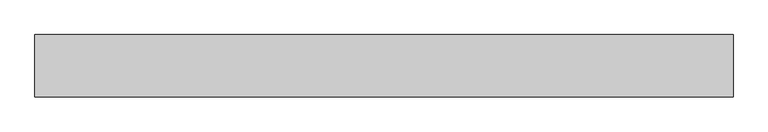
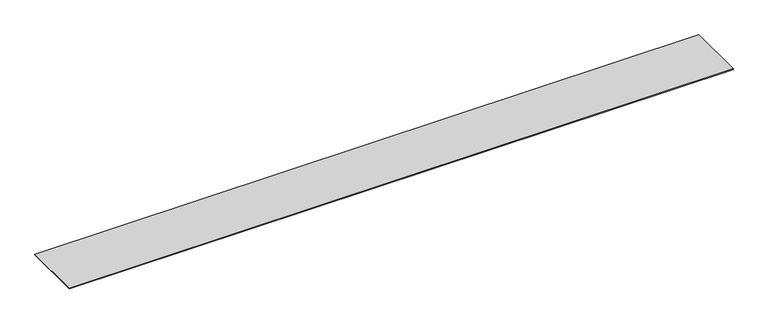
"""IFC4 building model written with IfcOpenShell, lengths in millimetres: proxy geometry, Generic Models 6:Generic Models 2:318829:Generic Models 2:318829 : Generic Models 6:Generic Models 2:318829:12 : Generic Models 6:Generic Models 2:318829:Generic Models 2:318829 : Generic Models 6:Generic Models 2:318829:300683."""

from ifc_helpers import new_model, si_unit, frame, origin, place, context, project, spatial, polyline, outline, extrude, source, transform, mapped, element, save


def generic_models_3f63b9cd(model_context):
    return source(origin(), model_context, "Body", "SweptSolid", [
        extrude(outline(polyline([(592755.4242239, -578871.8512905), (592755.4242239, -579089.5913841), (590317.0242239, -579089.5913841), (590317.0242239, -578871.8512905), (592755.4242239, -578871.8512905)])), frame((0.0, 0.0, 1.3315311), z_axis=(0.0, 0.0, 1.0), x_axis=(1.0, 0.0, 0.0)), (0.0, 0.0, 1.0), 2.3213461),
    ])


if __name__ == "__main__":
    model = new_model("IFC4")
    model_context = context("Model", 3, world=origin())
    ifc_project = project(units=[si_unit("LENGTHUNIT", "METRE", prefix="MILLI")], contexts=[model_context])
    site = spatial("IfcSite", under=ifc_project)
    building = spatial("IfcBuilding", under=site)
    placement = place(None, origin())
    generic_models_shape = generic_models_3f63b9cd(model_context)
    element("IfcBuildingElementProxy", 1, Name="Generic Models 6:Generic Models 2:318829:Generic Models 2:318829 : Generic Models 6:Generic Models 2:318829:12 : Generic Models 6:Generic Models 2:318829:Generic Models 2:318829 : Generic Models 6:Generic Models 2:318829:300683", ObjectType="Generic Models 6:Generic Models 2:318829:Generic Models 2:318829 : Generic Models 6:Generic Models 2:318829:12 : Generic Models 6:Generic Models 2:318829:Generic Models 2:318829 : Generic Models 6:Generic Models 2:318829:300683", at=placement, inside=building, context=model_context, shape_type="MappedRepresentation", body=[
        mapped(generic_models_shape, transform((0.0, 0.0, 0.0), x_axis=(1.0, 0.0, 0.0), y_axis=(0.0, 1.0, 0.0), z_axis=(0.0, 0.0, 1.0))),
    ])
    save(model, "model.ifc")

# Revit data of these elements
# Type "Generic Models 6:Generic Models 2:318829:Generic Models 2:318829 : Generic Models 6:Generic Models 2:318829:12 : Generic Models 6:Generic Models 2:318829:Generic Models 2:318829 : Generic Models 6:Generic Models 2:318829:300683"
#   NameOverride = "Generic Models 6:Generic Models 2:318829:Generic Models 2:318829 : Generic Models 6:Generic Models 2:318829:300683"
#   ObjectTypeOverride = "Generic Models 2:318829 : Generic Models 6:Generic Models 2:318829"
#   Reference = "Generic Models 2"
#   Tag = "300683"
# Element 1 (IfcBuildingElementProxy, "Generic Models 6:Generic Models 2:318829:Generic Models 2:318829 : Generic Models 6:Generic Models 2:318829:12 : Generic Models 6:Generic Models 2:318829:Generic Models 2:318829 : Generic Models 6:Generic Models 2:318829:300683")
#   Materials on its faces: "SILL GASKET"
# Materials
#   "SILL GASKET": class "Generic", colour RGB 160 254 137, transparency 0, Cost = 0
